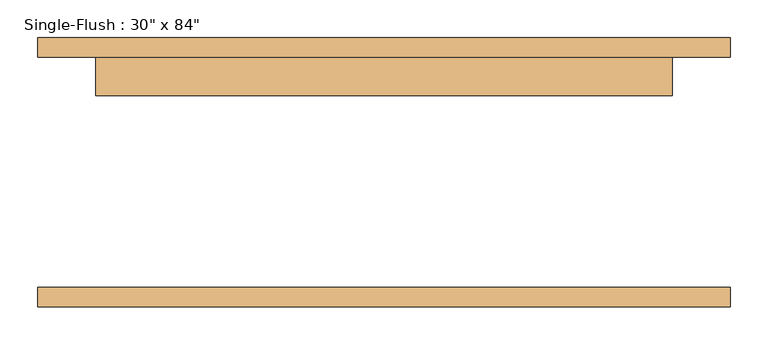
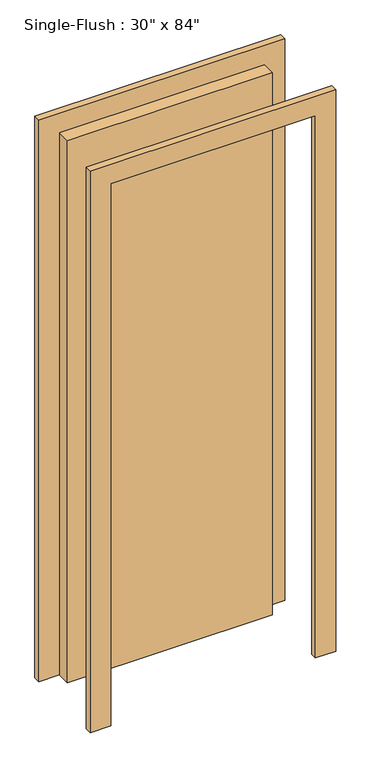
"""IFC4 building model written with IfcOpenShell, lengths in millimetres: door geometry."""

import ifcopenshell
import ifcopenshell.guid

model = None  # the IFC model being written
_history = None  # IfcOwnerHistory: only IFC2X3 demands one
_inside = {}  # id of a spatial element -> (the spatial element, [elements in it])
_under = {}  # id of a project, library or spatial element -> (it, [spatial elements below it])
_declared = {}  # id of a project -> (the project, [libraries it declares])
_typed = {}  # id of a type object -> (the type object, [elements of that type])
_made_of = {}  # id of a material, layer set ... -> (it, [elements and type objects made of it])


def new_model(schema):
    """Start an empty IFC model of exactly this schema.

    Asked for "IFC4X3", IfcOpenShell would pick the latest addendum, in which some entities
    have other attributes; the version numbers below select the first issue.
    IFC2X3 requires an IfcOwnerHistory on every rooted entity: one is made here for all.
    """
    global model, _history
    if schema == "IFC4X3":
        model = ifcopenshell.file(schema_version=(4, 3, 0, 0))
    else:
        model = ifcopenshell.file(schema=schema)
    _inside.clear()
    _under.clear()
    _declared.clear()
    _typed.clear()
    _made_of.clear()
    _history = None
    if model.schema == "IFC2X3":
        org = make("IfcOrganization", Name="unknown")
        user = make(
            "IfcPersonAndOrganization",
            ThePerson=make("IfcPerson", FamilyName="unknown"),
            TheOrganization=org,
        )
        app = make(
            "IfcApplication",
            ApplicationDeveloper=org,
            Version="unknown",
            ApplicationFullName="unknown",
            ApplicationIdentifier="unknown",
        )
        _history = make(
            "IfcOwnerHistory",
            OwningUser=user,
            OwningApplication=app,
            ChangeAction="ADDED",
            CreationDate=0,
        )
    return model


def make(cls, **values):
    """One entity of the class cls with the attributes given. An attribute that is None is left unset."""
    return model.create_entity(
        cls, **{name: value for name, value in values.items() if value is not None}
    )


def rooted(cls, **values):
    """An entity with a GlobalId (a new one), such as an element, a storey or a relation."""
    return make(cls, GlobalId=ifcopenshell.guid.new(), OwnerHistory=_history, **values)


def si_unit(unit_type, name, prefix=None):
    """IfcSIUnit, for example si_unit("LENGTHUNIT", "METRE", prefix="MILLI")."""
    return make("IfcSIUnit", UnitType=unit_type, Prefix=prefix, Name=name)


def assignment(units):
    """IfcUnitAssignment: the units of a project."""
    return None if units is None else make("IfcUnitAssignment", Units=units)


def point(xyz):
    """IfcCartesianPoint."""
    return None if xyz is None else make("IfcCartesianPoint", Coordinates=xyz)


def direction(xyz):
    """IfcDirection."""
    return None if xyz is None else make("IfcDirection", DirectionRatios=xyz)


def frame(location, z_axis=None, x_axis=None):
    """IfcAxis2Placement3D, a coordinate frame: its origin and axes. An axis left out is left unset."""
    return make(
        "IfcAxis2Placement3D",
        Location=point(location),
        Axis=direction(z_axis),
        RefDirection=direction(x_axis),
    )


def origin():
    """The frame at (0, 0, 0) with its axes left unset."""
    return frame((0.0, 0.0, 0.0))


def origin_with_axes():
    """The frame at (0, 0, 0) with the z axis (0, 0, 1) and the x axis (1, 0, 0) written out."""
    return frame((0.0, 0.0, 0.0), z_axis=(0.0, 0.0, 1.0), x_axis=(1.0, 0.0, 0.0))


def place(relative_to, where):
    """IfcLocalPlacement: puts the frame where relative to a parent placement (None: the world)."""
    return make(
        "IfcLocalPlacement", PlacementRelTo=relative_to, RelativePlacement=where
    )


def context(
    kind, dimensions, precision=None, world=None, true_north=None, identifier=None
):
    """IfcGeometricRepresentationContext, for example the 3D "Model" context."""
    return make(
        "IfcGeometricRepresentationContext",
        ContextIdentifier=identifier,
        ContextType=kind,
        CoordinateSpaceDimension=dimensions,
        Precision=precision,
        WorldCoordinateSystem=world,
        TrueNorth=true_north,
    )


def project(units=None, contexts=None):
    """IfcProject with its units and contexts."""
    return rooted(
        "IfcProject",
        Name="project",
        RepresentationContexts=contexts,
        UnitsInContext=assignment(units),
    )


def spatial(cls, under=None, at=None, **own):
    """A site, building, storey or space (cls), placed at a placement, below another one or the project."""
    s = rooted(cls, ObjectPlacement=at, **own)
    if under is not None:
        _under.setdefault(under.id(), (under, []))[1].append(s)
    return s


def polyline(points):
    """IfcPolyline through the points."""
    return make("IfcPolyline", Points=[point(p) for p in points])


def outline(outer, holes=None, kind="AREA"):
    """IfcArbitraryClosedProfileDef: a profile drawn as a closed curve; with holes, ...WithVoids."""
    if holes is None:
        return make("IfcArbitraryClosedProfileDef", ProfileType=kind, OuterCurve=outer)
    return make(
        "IfcArbitraryProfileDefWithVoids",
        ProfileType=kind,
        OuterCurve=outer,
        InnerCurves=holes,
    )


def extrude(swept, where, along, depth):
    """IfcExtrudedAreaSolid: the profile swept, set in the frame where, extruded along a direction by depth."""
    return make(
        "IfcExtrudedAreaSolid",
        SweptArea=swept,
        Position=where,
        ExtrudedDirection=direction(along),
        Depth=depth,
    )


def shape(context_of_items, identifier, shape_type, items):
    """IfcShapeRepresentation: the items that make up one representation, for example the "Body"."""
    return make(
        "IfcShapeRepresentation",
        ContextOfItems=context_of_items,
        RepresentationIdentifier=identifier,
        RepresentationType=shape_type,
        Items=items,
    )


def source(mapping_origin, context_of_items, identifier, shape_type, items):
    """IfcRepresentationMap: a shape defined once, which mapped items show again and again."""
    return make(
        "IfcRepresentationMap",
        MappingOrigin=mapping_origin,
        MappedRepresentation=shape(context_of_items, identifier, shape_type, items),
    )


def transform(
    local_origin,
    x_axis=None,
    y_axis=None,
    z_axis=None,
    scale=None,
    scale2=None,
    scale3=None,
    uniform=True,
):
    """IfcCartesianTransformationOperator3D, or its non-uniform kind. x_axis, y_axis, z_axis: its Axis1, 2, 3."""
    if uniform:
        return make(
            "IfcCartesianTransformationOperator3D",
            Axis1=direction(x_axis),
            Axis2=direction(y_axis),
            LocalOrigin=point(local_origin),
            Scale=scale,
            Axis3=direction(z_axis),
        )
    return make(
        "IfcCartesianTransformationOperator3DnonUniform",
        Axis1=direction(x_axis),
        Axis2=direction(y_axis),
        LocalOrigin=point(local_origin),
        Scale=scale,
        Axis3=direction(z_axis),
        Scale2=scale2,
        Scale3=scale3,
    )


def mapped(mapping_source, mapping_target):
    """IfcMappedItem: shows the shape of a source again, moved by a transform."""
    return make(
        "IfcMappedItem", MappingSource=mapping_source, MappingTarget=mapping_target
    )


def made_of(thing, what):
    """Note that an element or type object is made of a material, layer set ...; save() writes the relation."""
    if what is not None:
        _made_of.setdefault(what.id(), (what, []))[1].append(thing)
    return thing


def element(
    cls,
    number,
    at=None,
    inside=None,
    cuts=None,
    type_object=None,
    material=None,
    context=None,
    identifier="Body",
    shape_type=None,
    held_by="IfcProductDefinitionShape",
    body=None,
    shapes=None,
    **own,
):
    """One element of the class cls, such as IfcWall. Its Tag is "e" and its number.

    at: its placement. inside: the storey or other place that contains it. cuts: it is an
    opening in that element (IfcRelVoidsElement). A single representation is given by context,
    identifier, shape_type and body (its items); several are given by shapes. held_by: the class
    of the entity that holds the representations. save() writes the other relations.
    """
    e = rooted(cls, Tag="e%d" % number, ObjectPlacement=at, **own)
    if body is not None:
        shapes = [shape(context, identifier, shape_type, body)]
    if shapes is not None:
        e.Representation = make(held_by, Representations=shapes)
    if inside is not None:
        _inside.setdefault(inside.id(), (inside, []))[1].append(e)
    if cuts is not None:
        rooted(
            "IfcRelVoidsElement", RelatingBuildingElement=cuts, RelatedOpeningElement=e
        )
    if type_object is not None:
        _typed.setdefault(type_object.id(), (type_object, []))[1].append(e)
    return made_of(e, material)


def aggregate(whole, parts):
    """IfcRelAggregates: a whole, such as a stair, and the parts it consists of."""
    return rooted("IfcRelAggregates", RelatingObject=whole, RelatedObjects=parts)


def save(model, path):
    """Write the relations noted so far, then the file.

    IfcRelAggregates (storeys below a building ...), IfcRelContainedInSpatialStructure (elements
    in a storey), IfcRelDefinesByType, IfcRelAssociatesMaterial and IfcRelDeclares: one each for
    every whole, place, type object, material and project.
    """
    for whole, parts in _under.values():
        aggregate(whole, parts)
    for where, things in _inside.values():
        rooted(
            "IfcRelContainedInSpatialStructure",
            RelatedElements=things,
            RelatingStructure=where,
        )
    for kind, things in _typed.values():
        rooted("IfcRelDefinesByType", RelatedObjects=things, RelatingType=kind)
    for what, things in _made_of.values():
        rooted("IfcRelAssociatesMaterial", RelatedObjects=things, RelatingMaterial=what)
    for by, libraries in _declared.values():
        rooted("IfcRelDeclares", RelatingContext=by, RelatedDefinitions=libraries)
    model.write(path)


def door_fd98f027(model_context):
    return source(origin(), model_context, "Body", "SweptSolid", [
        extrude(outline(polyline([(2209.8, -457.2), (0.0, -457.2), (0.0, -381.0), (2133.6, -381.0), (2133.6, 381.0), (0.0, 381.0), (0.0, 457.2), (2209.8, 457.2), (2209.8, -457.2)])), frame((0.0, 152.4, 0.0), z_axis=(0.0, 1.0, 0.0), x_axis=(0.0, 0.0, 1.0)), (0.0, 0.0, 1.0), 25.4),
        extrude(outline(polyline([(2209.8, 457.2), (2209.8, -457.2), (0.0, -457.2), (0.0, -381.0), (2133.6, -381.0), (2133.6, 381.0), (0.0, 381.0), (0.0, 457.2), (2209.8, 457.2)])), frame((0.0, -177.8, 0.0), z_axis=(0.0, 1.0, 0.0), x_axis=(0.0, 0.0, 1.0)), (0.0, 0.0, 1.0), 25.4),
        extrude(outline(polyline([(381.0, 101.6), (-381.0, 101.6), (-381.0, 152.4), (381.0, 152.4), (381.0, 101.6)])), origin_with_axes(), (0.0, 0.0, 1.0), 2133.6),
    ])


if __name__ == "__main__":
    model = new_model("IFC4")
    model_context = context("Model", 3, world=origin())
    ifc_project = project(units=[si_unit("LENGTHUNIT", "METRE", prefix="MILLI")], contexts=[model_context])
    site = spatial("IfcSite", under=ifc_project)
    building = spatial("IfcBuilding", under=site)
    placement = place(None, origin())
    door_shape = door_fd98f027(model_context)
    element("IfcDoor", 1, ObjectType="Single-Flush : 30\" x 84\"", at=placement, inside=building, context=model_context, shape_type="MappedRepresentation", body=[
        mapped(door_shape, transform((0.0, 0.0, 0.0), x_axis=(1.0, 0.0, 0.0), y_axis=(0.0, 1.0, 0.0), z_axis=(0.0, 0.0, 1.0))),
    ])
    save(model, "model.ifc")

# Revit data of these elements
# Type "Single-Flush : 30\" x 84\""
#   Type Mark = "4"
#   Construction Type Id = "MDOOR"
#   Assembly Code = "C1020"
#   Analytic Construction = "Metal"
#   Thickness = 0' - 2"
#   Heat Transfer Coefficient (U) = 0.651978 BTU/(h·ft²·°F)
#   Height = 7' - 0"
#   Trim Projection Ext = 0' - 1"
#   Trim Projection Int = 0' - 1"
#   Trim Width = 0' - 3"
#   Width = 2' - 6"
#   Define Thermal Properties by = 1
#   Define Thermal Properties by = 1
#   Door Material = Door - Panel
#   Frame Material = Door - Frame
#   Visual Light Transmittance = 0
#   Solar Heat Gain Coefficient = 0
#   Function = (empty or 0)
#   Wall Closure = (empty or 0)
# Element 1 (IfcDoor, "Single-Flush : 30\" x 84\"")
#   Materials on its faces: "Door - Frame", "Door - Panel"
# Materials
#   "Door - Panel": class "Wood", colour RGB 210 159 95, transparency 0, Cost = 0
#   "Door - Frame": class "Miscellaneous", colour RGB 118 70 51, transparency 0, Cost = 0
